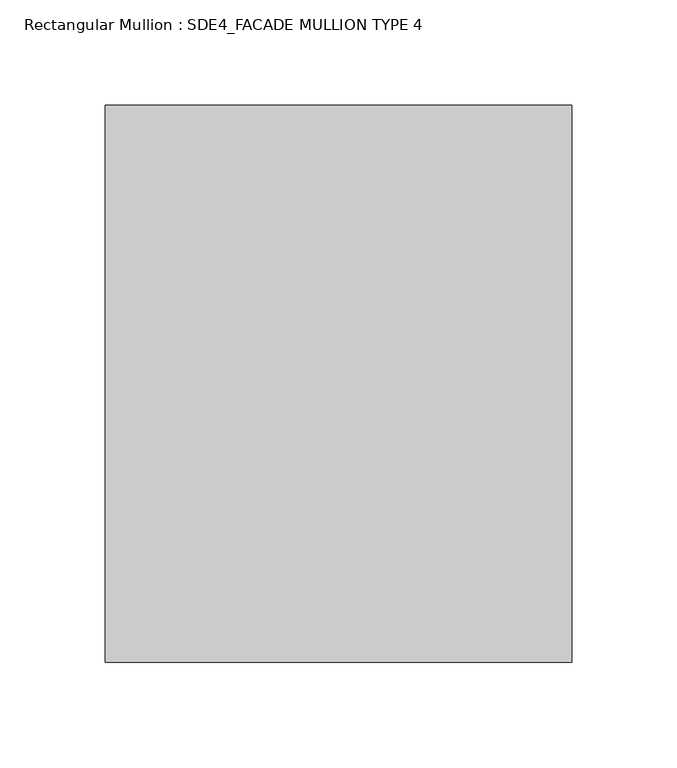
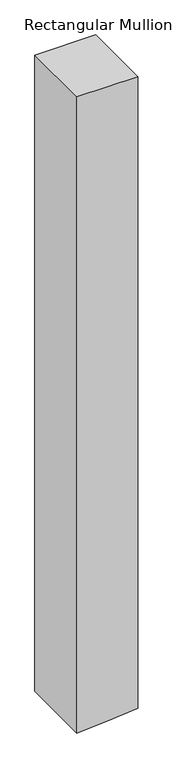
"""IFC4 building model written with IfcOpenShell, lengths in millimetres: member geometry, Rectangular Mullion : SDE4_FACADE MULLION TYPE 4."""

from ifc_helpers import new_model, si_unit, frame, origin, place, context, project, spatial, polyline, outline, extrude, source, transform, mapped, element, save


def rectangular_mullion_sde4_facade_mullion_type_4_a6836284(model_context):
    return source(origin(), model_context, "Body", "SweptSolid", [
        extrude(outline(polyline([(0.0, 111.0), (0.0, -111.0), (-2448.8743823, -111.0), (-2440.6019424, -3.056508), (-2431.8610208, 111.0), (0.0, 111.0)])), frame((0.0, -132.5, 0.0), z_axis=(0.0, 1.0, 0.0), x_axis=(0.0, 0.0, 1.0)), (0.0, 0.0, 1.0), 265.0),
    ])


if __name__ == "__main__":
    model = new_model("IFC4")
    model_context = context("Model", 3, world=origin())
    ifc_project = project(units=[si_unit("LENGTHUNIT", "METRE", prefix="MILLI")], contexts=[model_context])
    site = spatial("IfcSite", under=ifc_project)
    building = spatial("IfcBuilding", under=site)
    placement = place(None, origin())
    rectangular_mullion_sde4_facade_mullion_type_4_shape = rectangular_mullion_sde4_facade_mullion_type_4_a6836284(model_context)
    element("IfcMember", 1, ObjectType="Rectangular Mullion : SDE4_FACADE MULLION TYPE 4", at=placement, inside=building, context=model_context, shape_type="MappedRepresentation", body=[
        mapped(rectangular_mullion_sde4_facade_mullion_type_4_shape, transform((0.0, 0.0, 0.0), x_axis=(1.0, 0.0, 0.0), y_axis=(0.0, 1.0, 0.0), z_axis=(0.0, 0.0, 1.0))),
    ])
    save(model, "model.ifc")

# Revit data of these elements
# Type "Rectangular Mullion : SDE4_FACADE MULLION TYPE 4"
#   built-in parameter 1007322 = 0.869423 (stored number, unit not read)
#   built-in parameter 1007321 = 0.364173 (stored number, unit not read)
#   built-in parameter 1007320 = 0.364173 (stored number, unit not read)
